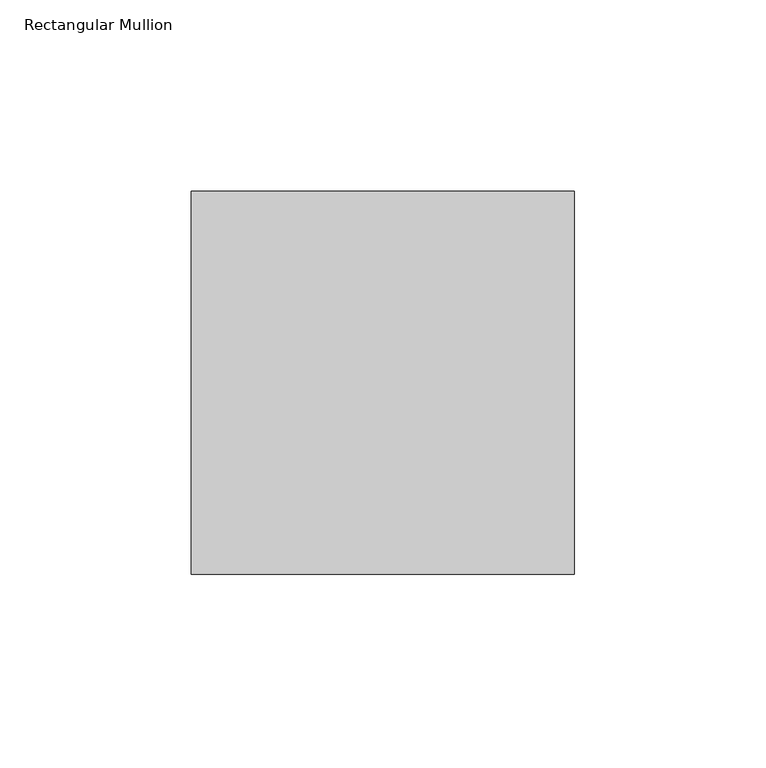
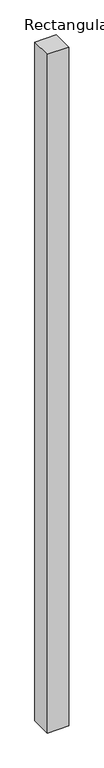
"""IFC4 building model written with IfcOpenShell, lengths in millimetres: member geometry, Rectangular Mullion : 알루미늄_Rectangular Cap_100 x100."""

from ifc_helpers import new_model, si_unit, frame, origin, place, context, project, spatial, polyline, outline, extrude, source, transform, mapped, element, save


def rectangular_mullion_9dbe7c8d(model_context):
    return source(origin(), model_context, "Body", "SweptSolid", [
        extrude(outline(polyline([(0.0, 50.0), (0.0, -50.0), (-100.0, -50.0), (-100.0, 50.0), (0.0, 50.0)])), frame((0.0, 0.0, -3325.0), z_axis=(0.0, 0.0, 1.0), x_axis=(1.0, 0.0, 0.0)), (0.0, 0.0, 1.0), 3325.0),
    ])


if __name__ == "__main__":
    model = new_model("IFC4")
    model_context = context("Model", 3, world=origin())
    ifc_project = project(units=[si_unit("LENGTHUNIT", "METRE", prefix="MILLI")], contexts=[model_context])
    site = spatial("IfcSite", under=ifc_project)
    building = spatial("IfcBuilding", under=site)
    placement = place(None, origin())
    rectangular_mullion_shape = rectangular_mullion_9dbe7c8d(model_context)
    element("IfcMember", 1, ObjectType="Rectangular Mullion : 알루미늄_Rectangular Cap_100 x100", at=placement, inside=building, context=model_context, shape_type="MappedRepresentation", body=[
        mapped(rectangular_mullion_shape, transform((0.0, 0.0, 0.0), x_axis=(1.0, 0.0, 0.0), y_axis=(0.0, 1.0, 0.0), z_axis=(0.0, 0.0, 1.0))),
    ])
    save(model, "model.ifc")

# Revit data of these elements
# Type "Rectangular Mullion : 알루미늄_Rectangular Cap_100 x100"
#   built-in parameter 1007304 = 0.328084 (stored number, unit not read)
#   built-in parameter 1007301 = 0.164042 (stored number, unit not read)
#   built-in parameter 1007300 = 0.164042 (stored number, unit not read)
# Element 1 (IfcMember, "Rectangular Mullion : 알루미늄_Rectangular Cap_100 x100")
#   Materials on its faces: "00_Metal_Stainless Steel"
# Materials
#   "00_Metal_Stainless Steel": class "Metal", colour RGB 148 148 148, transparency 0, Description = "Steel", Cost = 0
